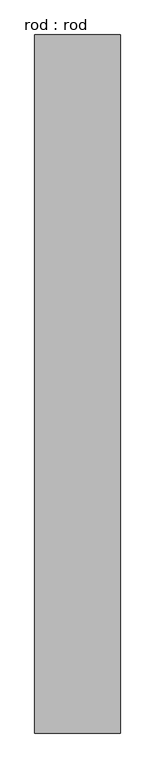
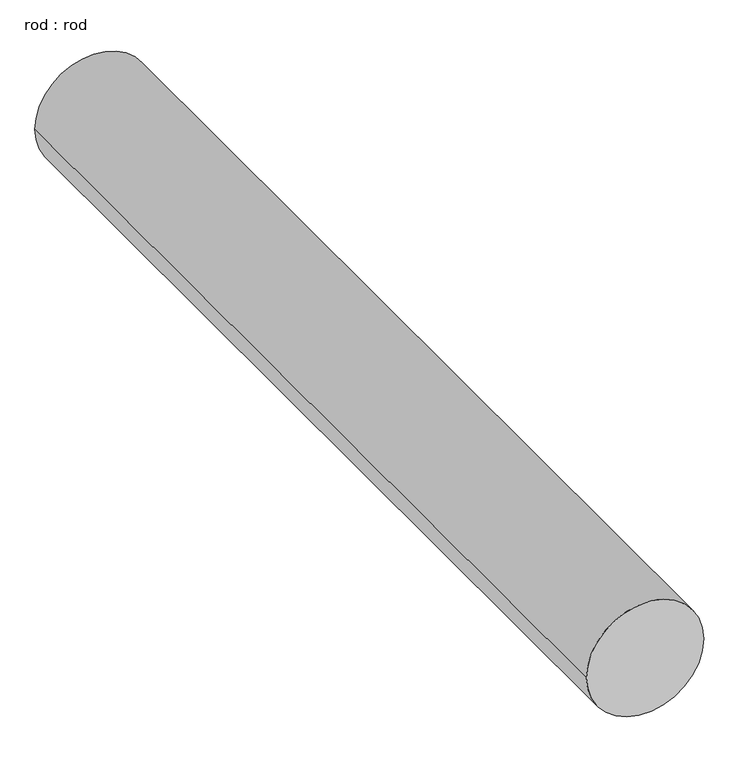
"""IFC4 building model written with IfcOpenShell, lengths in millimetres: proxy geometry, rod : rod."""

from ifc_helpers import new_model, si_unit, point, frame, frame_2d, origin, place, context, project, spatial, circle_curve, trimmed, segment, composite_curve, outline, extrude, source, transform, mapped, element, save


def rod_rod_d847fa41(model_context):
    return source(origin(), model_context, "Body", "SweptSolid", [
        extrude(outline(composite_curve([segment(trimmed(circle_curve(frame_2d((0.0108462, 0.0)), 200.0), [point((0.0108462, 200.0))], [point((0.0108462, -200.0))], False, "CARTESIAN"), True, "CONTINUOUS"), segment(trimmed(circle_curve(frame_2d((0.0108462, 0.0)), 200.0), [point((0.0108462, -200.0))], [point((0.0108462, 200.0))], False, "CARTESIAN"), True, "CONTINUOUS")], self_intersect=False)), frame((0.0, 2462.7286153, 0.0), z_axis=(0.0, 1.0, 0.0), x_axis=(0.0, 0.0, 1.0)), (0.0, 0.0, 1.0), 3260.0),
    ])


if __name__ == "__main__":
    model = new_model("IFC4")
    model_context = context("Model", 3, world=origin())
    ifc_project = project(units=[si_unit("LENGTHUNIT", "METRE", prefix="MILLI")], contexts=[model_context])
    site = spatial("IfcSite", under=ifc_project)
    building = spatial("IfcBuilding", under=site)
    placement = place(None, origin())
    rod_rod_shape = rod_rod_d847fa41(model_context)
    element("IfcBuildingElementProxy", 1, Name="rod : rod", ObjectType="rod : rod", at=placement, inside=building, context=model_context, shape_type="MappedRepresentation", body=[
        mapped(rod_rod_shape, transform((0.0, 0.0, 0.0), x_axis=(1.0, 0.0, 0.0), y_axis=(0.0, 1.0, 0.0), z_axis=(0.0, 0.0, 1.0))),
    ])
    save(model, "model.ifc")

# Revit data of these elements
# Type "rod : rod"
#   Default Elevation = 0
